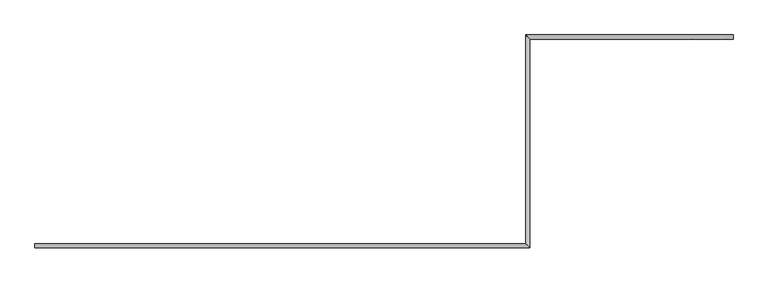
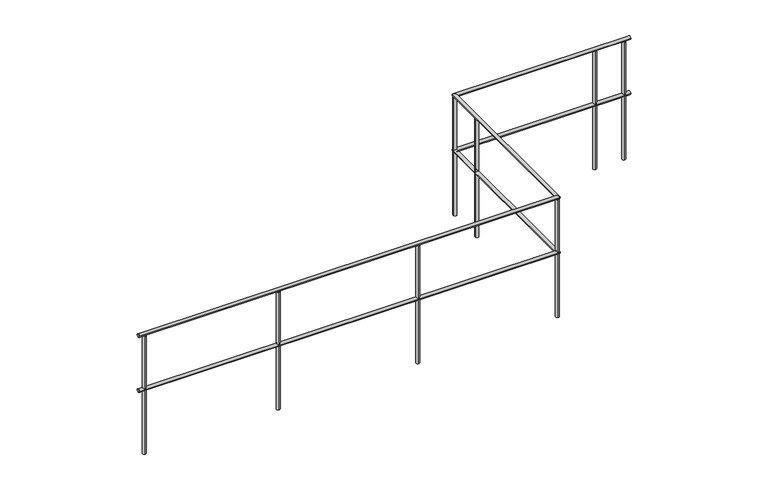
"""IFC4 building model written with IfcOpenShell, lengths in millimetres: railing geometry."""

from ifc_helpers import new_model, si_unit, point, frame, frame_2d, origin, place, context, project, spatial, circle_curve, ellipse_curve, trimmed, segment, composite_curve, outline, extrude, source, transform, mapped, element, save
from ifc_brep_helpers import plane_surface, cylinder_surface, advanced_brep


def railing_814e4083(model_context):
    return source(origin(), model_context, "Body", "SolidModel", [
        advanced_brep(
        [(60716.32048, 71467.0208589, 885.0), (60716.32048, 71437.0208589, 885.0), (64301.0, 71467.0208589, 885.0), (64331.0, 71437.0208589, 885.0), (64301.0, 72992.0208589, 885.0), (64331.0, 72962.0208589, 885.0), (65816.3017909, 72992.0208589, 885.0), (65816.3017909, 72962.0208589, 885.0)],
        [
            (0, 1, circle_curve(frame((60716.32048, 71452.0208589, 885.0), z_axis=(-1.0, 0.0, 0.0), x_axis=(0.0, -1.0, 0.0)), 15.0)),
            (1, 0, circle_curve(frame((60716.32048, 71452.0208589, 885.0), z_axis=(-1.0, 0.0, 0.0), x_axis=(0.0, -1.0, 0.0)), 15.0)),
            (0, 2),
            (2, 3, ellipse_curve(frame((64316.0, 71452.0208589, 885.0), z_axis=(-0.7071067811865483, -0.7071067811865466, 0.0), x_axis=(-0.7071067811865467, 0.7071067811865482, 0.0)), 21.2132034, 15.0)),
            (3, 1),
            (3, 2, ellipse_curve(frame((64316.0, 71452.0208589, 885.0), z_axis=(-0.7071067811865483, -0.7071067811865466, 0.0), x_axis=(-0.7071067811865467, 0.7071067811865482, 0.0)), 21.2132034, 15.0)),
            (2, 4),
            (4, 5, ellipse_curve(frame((64316.0, 72977.0208589, 885.0), z_axis=(-0.7071067811865496, -0.7071067811865455, 0.0), x_axis=(0.7071067811865455, -0.7071067811865496, 0.0)), 21.2132034, 15.0)),
            (5, 3),
            (5, 4, ellipse_curve(frame((64316.0, 72977.0208589, 885.0), z_axis=(-0.7071067811865496, -0.7071067811865455, 0.0), x_axis=(0.7071067811865455, -0.7071067811865496, 0.0)), 21.2132034, 15.0)),
            (6, 7, circle_curve(frame((65816.3017909, 72977.0208589, 885.0), z_axis=(1.0, 0.0, 0.0), x_axis=(0.0, -1.0, 0.0)), 15.0)),
            (7, 6, circle_curve(frame((65816.3017909, 72977.0208589, 885.0), z_axis=(1.0, 0.0, 0.0), x_axis=(0.0, -1.0, 0.0)), 15.0)),
            (4, 6),
            (7, 5),
        ],
        [
            plane_surface(frame((60716.32048, 71452.0208589, 900.0), z_axis=(-1.0, 0.0, 0.0), x_axis=(0.0, 1.0, 0.0))),
            cylinder_surface(frame((60716.32048, 71452.0208589, 885.0), z_axis=(-1.0, 0.0, 0.0), x_axis=(0.0, -1.0, 0.0)), 15.0),
            cylinder_surface(frame((64316.0, 71452.0208589, 885.0), z_axis=(0.0, -1.0, 0.0), x_axis=(1.0, 0.0, 0.0)), 15.0),
            plane_surface(frame((65816.3017909, 72977.0208589, 900.0), z_axis=(1.0, 0.0, 0.0), x_axis=(0.0, 1.0, 0.0))),
            cylinder_surface(frame((64316.0, 72977.0208589, 885.0), z_axis=(-1.0, 0.0, 0.0), x_axis=(0.0, -1.0, 0.0)), 15.0),
        ],
        [
            (0, [[1, 2]]),
            (1, [[-1, 3, 4, 5]]),
            (1, [[-2, -5, 6, -3]]),
            (2, [[-4, 7, 8, 9]]),
            (2, [[-6, -9, 10, -7]]),
            (3, [[11, 12]]),
            (4, [[-8, 13, -12, 14]]),
            (4, [[-10, -14, -11, -13]]),
        ],
    ),
        advanced_brep(
        [(60716.32048, 71467.0208589, 1385.0), (60716.32048, 71437.0208589, 1385.0), (64301.0, 71467.0208589, 1385.0), (64331.0, 71437.0208589, 1385.0), (64301.0, 72992.0208589, 1385.0), (64331.0, 72962.0208589, 1385.0), (65816.3017909, 72992.0208589, 1385.0), (65816.3017909, 72962.0208589, 1385.0)],
        [
            (0, 1, circle_curve(frame((60716.32048, 71452.0208589, 1385.0), z_axis=(-1.0, 0.0, 0.0), x_axis=(0.0, -1.0, 0.0)), 15.0)),
            (1, 0, circle_curve(frame((60716.32048, 71452.0208589, 1385.0), z_axis=(-1.0, 0.0, 0.0), x_axis=(0.0, -1.0, 0.0)), 15.0)),
            (0, 2),
            (2, 3, ellipse_curve(frame((64316.0, 71452.0208589, 1385.0), z_axis=(-0.7071067811865483, -0.7071067811865466, 0.0), x_axis=(-0.7071067811865467, 0.7071067811865482, 0.0)), 21.2132034, 15.0)),
            (3, 1),
            (3, 2, ellipse_curve(frame((64316.0, 71452.0208589, 1385.0), z_axis=(-0.7071067811865483, -0.7071067811865466, 0.0), x_axis=(-0.7071067811865467, 0.7071067811865482, 0.0)), 21.2132034, 15.0)),
            (2, 4),
            (4, 5, ellipse_curve(frame((64316.0, 72977.0208589, 1385.0), z_axis=(-0.7071067811865496, -0.7071067811865455, 0.0), x_axis=(0.7071067811865455, -0.7071067811865496, 0.0)), 21.2132034, 15.0)),
            (5, 3),
            (5, 4, ellipse_curve(frame((64316.0, 72977.0208589, 1385.0), z_axis=(-0.7071067811865496, -0.7071067811865455, 0.0), x_axis=(0.7071067811865455, -0.7071067811865496, 0.0)), 21.2132034, 15.0)),
            (6, 7, circle_curve(frame((65816.3017909, 72977.0208589, 1385.0), z_axis=(1.0, 0.0, 0.0), x_axis=(0.0, -1.0, 0.0)), 15.0)),
            (7, 6, circle_curve(frame((65816.3017909, 72977.0208589, 1385.0), z_axis=(1.0, 0.0, 0.0), x_axis=(0.0, -1.0, 0.0)), 15.0)),
            (4, 6),
            (7, 5),
        ],
        [
            plane_surface(frame((60716.32048, 71452.0208589, 1400.0), z_axis=(-1.0, 0.0, 0.0), x_axis=(0.0, 1.0, 0.0))),
            cylinder_surface(frame((60716.32048, 71452.0208589, 1385.0), z_axis=(-1.0, 0.0, 0.0), x_axis=(0.0, -1.0, 0.0)), 15.0),
            cylinder_surface(frame((64316.0, 71452.0208589, 1385.0), z_axis=(0.0, -1.0, 0.0), x_axis=(1.0, 0.0, 0.0)), 15.0),
            plane_surface(frame((65816.3017909, 72977.0208589, 1400.0), z_axis=(1.0, 0.0, 0.0), x_axis=(0.0, 1.0, 0.0))),
            cylinder_surface(frame((64316.0, 72977.0208589, 1385.0), z_axis=(-1.0, 0.0, 0.0), x_axis=(0.0, -1.0, 0.0)), 15.0),
        ],
        [
            (0, [[1, 2]]),
            (1, [[-1, 3, 4, 5]]),
            (1, [[-2, -5, 6, -3]]),
            (2, [[-4, 7, 8, 9]]),
            (2, [[-6, -9, 10, -7]]),
            (3, [[11, 12]]),
            (4, [[-8, 13, -12, 14]]),
            (4, [[-10, -14, -11, -13]]),
        ],
    ),
        extrude(outline(composite_curve([segment(trimmed(circle_curve(frame_2d((65516.0, 72977.0208589)), 15.0), [point((65516.0, 72992.0208589))], [point((65516.0, 72962.0208589))], False, "CARTESIAN"), True, "CONTINUOUS"), segment(trimmed(circle_curve(frame_2d((65516.0, 72977.0208589)), 15.0), [point((65516.0, 72962.0208589))], [point((65516.0, 72992.0208589))], False, "CARTESIAN"), True, "CONTINUOUS")], self_intersect=False)), frame((0.0, 0.0, 300.0), z_axis=(0.0, 0.0, 1.0), x_axis=(1.0, 0.0, 0.0)), (0.0, 0.0, 1.0), 1070.0),
        extrude(outline(composite_curve([segment(trimmed(circle_curve(frame_2d((64316.0, 72652.0208589)), 15.0), [point((64301.0, 72652.0208589))], [point((64331.0, 72652.0208589))], False, "CARTESIAN"), True, "CONTINUOUS"), segment(trimmed(circle_curve(frame_2d((64316.0, 72652.0208589)), 15.0), [point((64331.0, 72652.0208589))], [point((64301.0, 72652.0208589))], False, "CARTESIAN"), True, "CONTINUOUS")], self_intersect=False)), frame((0.0, 0.0, 300.0), z_axis=(0.0, 0.0, 1.0), x_axis=(1.0, 0.0, 0.0)), (0.0, 0.0, 1.0), 1070.0),
        extrude(outline(composite_curve([segment(trimmed(circle_curve(frame_2d((63116.32048, 71452.0208589)), 15.0), [point((63116.32048, 71467.0208589))], [point((63116.32048, 71437.0208589))], False, "CARTESIAN"), True, "CONTINUOUS"), segment(trimmed(circle_curve(frame_2d((63116.32048, 71452.0208589)), 15.0), [point((63116.32048, 71437.0208589))], [point((63116.32048, 71467.0208589))], False, "CARTESIAN"), True, "CONTINUOUS")], self_intersect=False)), frame((0.0, 0.0, 300.0), z_axis=(0.0, 0.0, 1.0), x_axis=(1.0, 0.0, 0.0)), (0.0, 0.0, 1.0), 1070.0),
        extrude(outline(composite_curve([segment(trimmed(circle_curve(frame_2d((61916.32048, 71452.0208589)), 15.0), [point((61916.32048, 71467.0208589))], [point((61916.32048, 71437.0208589))], False, "CARTESIAN"), True, "CONTINUOUS"), segment(trimmed(circle_curve(frame_2d((61916.32048, 71452.0208589)), 15.0), [point((61916.32048, 71437.0208589))], [point((61916.32048, 71467.0208589))], False, "CARTESIAN"), True, "CONTINUOUS")], self_intersect=False)), frame((0.0, 0.0, 300.0), z_axis=(0.0, 0.0, 1.0), x_axis=(1.0, 0.0, 0.0)), (0.0, 0.0, 1.0), 1070.0),
        extrude(outline(composite_curve([segment(trimmed(circle_curve(frame_2d((64316.0, 72977.0208589)), 15.0), [point((64301.0, 72977.0208589))], [point((64331.0, 72977.0208589))], False, "CARTESIAN"), True, "CONTINUOUS"), segment(trimmed(circle_curve(frame_2d((64316.0, 72977.0208589)), 15.0), [point((64331.0, 72977.0208589))], [point((64301.0, 72977.0208589))], False, "CARTESIAN"), True, "CONTINUOUS")], self_intersect=False)), frame((0.0, 0.0, 300.0), z_axis=(0.0, 0.0, 1.0), x_axis=(1.0, 0.0, 0.0)), (0.0, 0.0, 1.0), 1070.0),
        extrude(outline(composite_curve([segment(trimmed(circle_curve(frame_2d((64316.0, 71452.0208589)), 15.0), [point((64316.0, 71467.0208589))], [point((64316.0, 71437.0208589))], False, "CARTESIAN"), True, "CONTINUOUS"), segment(trimmed(circle_curve(frame_2d((64316.0, 71452.0208589)), 15.0), [point((64316.0, 71437.0208589))], [point((64316.0, 71467.0208589))], False, "CARTESIAN"), True, "CONTINUOUS")], self_intersect=False)), frame((0.0, 0.0, 300.0), z_axis=(0.0, 0.0, 1.0), x_axis=(1.0, 0.0, 0.0)), (0.0, 0.0, 1.0), 1070.0),
        extrude(outline(composite_curve([segment(trimmed(circle_curve(frame_2d((65766.3017909, 72977.0208589)), 15.0), [point((65766.3017909, 72992.0208589))], [point((65766.3017909, 72962.0208589))], False, "CARTESIAN"), True, "CONTINUOUS"), segment(trimmed(circle_curve(frame_2d((65766.3017909, 72977.0208589)), 15.0), [point((65766.3017909, 72962.0208589))], [point((65766.3017909, 72992.0208589))], False, "CARTESIAN"), True, "CONTINUOUS")], self_intersect=False)), frame((0.0, 0.0, 300.0), z_axis=(0.0, 0.0, 1.0), x_axis=(1.0, 0.0, 0.0)), (0.0, 0.0, 1.0), 1070.0),
        extrude(outline(composite_curve([segment(trimmed(circle_curve(frame_2d((60766.32048, 71452.0208589)), 15.0), [point((60766.32048, 71467.0208589))], [point((60766.32048, 71437.0208589))], False, "CARTESIAN"), True, "CONTINUOUS"), segment(trimmed(circle_curve(frame_2d((60766.32048, 71452.0208589)), 15.0), [point((60766.32048, 71437.0208589))], [point((60766.32048, 71467.0208589))], False, "CARTESIAN"), True, "CONTINUOUS")], self_intersect=False)), frame((0.0, 0.0, 300.0), z_axis=(0.0, 0.0, 1.0), x_axis=(1.0, 0.0, 0.0)), (0.0, 0.0, 1.0), 1070.0),
    ])


if __name__ == "__main__":
    model = new_model("IFC4")
    model_context = context("Model", 3, world=origin())
    ifc_project = project(units=[si_unit("LENGTHUNIT", "METRE", prefix="MILLI")], contexts=[model_context])
    site = spatial("IfcSite", under=ifc_project)
    building = spatial("IfcBuilding", under=site)
    placement = place(None, origin())
    railing_shape = railing_814e4083(model_context)
    element("IfcRailing", 1, at=placement, inside=building, context=model_context, shape_type="MappedRepresentation", body=[
        mapped(railing_shape, transform((0.0, 0.0, 0.0), x_axis=(1.0, 0.0, 0.0), y_axis=(0.0, 1.0, 0.0), z_axis=(0.0, 0.0, 1.0))),
    ])
    save(model, "model.ifc")
